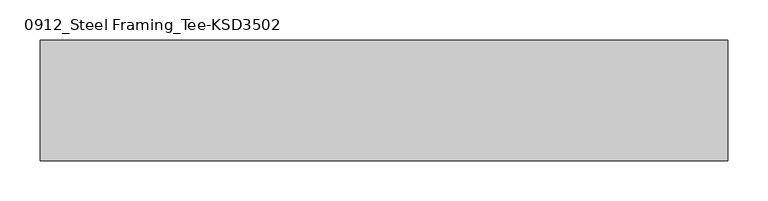
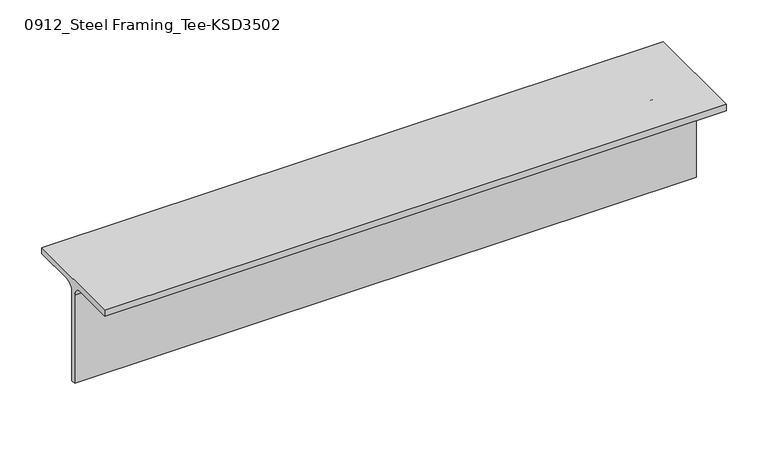
"""IFC4 building model written with IfcOpenShell, lengths in millimetres: member geometry, 0912_Steel Framing_Tee-KSD3502 : H_SB_ASB_CT-150x150x6.5x9."""

from ifc_helpers import new_model, si_unit, point, frame, frame_2d, origin, place, context, project, spatial, polyline, circle_curve, trimmed, segment, composite_curve, outline, extrude, source, transform, mapped, element, save


def member_0912_steel_framing_tee_ksd3502_f59be032(model_context):
    return source(origin(), model_context, "Body", "SweptSolid", [
        extrude(outline(composite_curve([segment(polyline([(75.0, 75.0), (75.0, 66.0), (16.25, 66.0)]), True, "CONTINUOUS"), segment(trimmed(circle_curve(frame_2d((16.25, 53.0)), 13.0), [point((16.25, 66.0))], [point((3.25, 53.0))], True, "CARTESIAN"), True, "CONTINUOUS"), segment(polyline([(3.25, 53.0), (3.25, -75.0), (-3.25, -75.0), (-3.25, 53.0)]), True, "CONTINUOUS"), segment(trimmed(circle_curve(frame_2d((-16.25, 53.0)), 13.0), [point((-3.25, 53.0))], [point((-16.25, 66.0))], True, "CARTESIAN"), True, "CONTINUOUS"), segment(polyline([(-16.25, 66.0), (-75.0, 66.0), (-75.0, 75.0), (75.0, 75.0)]), True, "CONTINUOUS")], self_intersect=False)), frame((-356.1, 0.0, 0.0), z_axis=(1.0, 0.0, 0.0), x_axis=(0.0, 1.0, 0.0)), (0.0, 0.0, 1.0), 856.1),
    ])


if __name__ == "__main__":
    model = new_model("IFC4")
    model_context = context("Model", 3, world=origin())
    ifc_project = project(units=[si_unit("LENGTHUNIT", "METRE", prefix="MILLI")], contexts=[model_context])
    site = spatial("IfcSite", under=ifc_project)
    building = spatial("IfcBuilding", under=site)
    placement = place(None, origin())
    member_0912_steel_framing_tee_ksd3502_shape = member_0912_steel_framing_tee_ksd3502_f59be032(model_context)
    element("IfcMember", 1, ObjectType="0912_Steel Framing_Tee-KSD3502 : H_SB_ASB_CT-150x150x6.5x9", at=placement, inside=building, context=model_context, shape_type="MappedRepresentation", body=[
        mapped(member_0912_steel_framing_tee_ksd3502_shape, transform((0.0, 0.0, 0.0), x_axis=(1.0, 0.0, 0.0), y_axis=(0.0, 1.0, 0.0), z_axis=(0.0, 0.0, 1.0))),
    ])
    save(model, "model.ifc")

# Revit data of these elements
# Type "0912_Steel Framing_Tee-KSD3502 : H_SB_ASB_CT-150x150x6.5x9"
#   H_WM Code_1 = "S01AA003-00001 | Main Steel Structure Fabrication Work | Shelter/Building | Light Steel - Standard (30KG/M>Weight) | Material: (   )"
#   H_WM Code_2 = "S03AA029-00001 | Main Steel Structure Erection Work | Shelter/Building | Light Steel (30KG/M>Weight) | Material: (   )"
#   H_WM Code_3 = "S01AA010-00001 | Main Steel Structure Fabrication Work | Shelter/Building | Steel Painting/Coating | for Non-Fireproofed Steel Surface, Surface Preparation, Primer, Second & Final Coat | Material: (   )"
#   H_Q'ty Cal Type Tag = "SB-Q2"
#   Width = 15.0 cm
#   Web Thickness = 0.65 cm
#   Web Fillet = 1.3 cm
#   Section Area = 23.39 cm²
#   Perimeter = 0.60 m²/m
#   Nominal Weight = 18.40 kgf/m
#   Height = 15.0 cm
#   Flange Thickness = 0.9 cm
#   Centroid Vertical = 7.5 cm
#   Centroid Horizontal = 7.5 cm
#   Length [instance default] = 1.5000 m
#   Structural Material [instance default] = Steel, 45-345
#   Warping Constant = (empty or 0)
#   Torsional Moment of Inertia = 0
#   Section Name Key = ""
#   Plastic Modulus weak axis = 0
#   Plastic Modulus strong axis = 0
#   Moment of Inertia weak axis = 0
#   Moment of Inertia strong axis = 0
#   Elastic Modulus weak axis = 0
#   Elastic Modulus strong axis = 0
#   Bolt Spacing = 0
#   Assembly Code = ""
# Element 1 (IfcMember, "0912_Steel Framing_Tee-KSD3502 : H_SB_ASB_CT-150x150x6.5x9")
#   Structural Material = none
# Materials
#   "Steel, 45-345": class "Metal", colour RGB 189 187 185, transparency 0, Description = "Steel 345 MPa", Cost = 0
